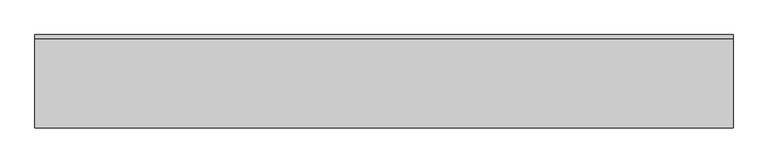
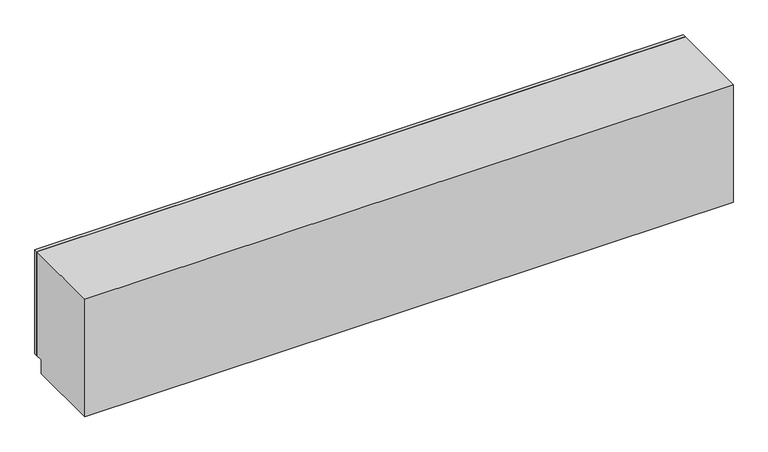
"""IFC4 building model written with IfcOpenShell, lengths in millimetres: furniture geometry, OD_CW_Base Cabinet : OD_CW_Base Cabinet."""

import ifcopenshell
import ifcopenshell.guid

model = None  # the IFC model being written
_history = None  # IfcOwnerHistory: only IFC2X3 demands one
_inside = {}  # id of a spatial element -> (the spatial element, [elements in it])
_under = {}  # id of a project, library or spatial element -> (it, [spatial elements below it])
_declared = {}  # id of a project -> (the project, [libraries it declares])
_typed = {}  # id of a type object -> (the type object, [elements of that type])
_made_of = {}  # id of a material, layer set ... -> (it, [elements and type objects made of it])


def new_model(schema):
    """Start an empty IFC model of exactly this schema.

    Asked for "IFC4X3", IfcOpenShell would pick the latest addendum, in which some entities
    have other attributes; the version numbers below select the first issue.
    IFC2X3 requires an IfcOwnerHistory on every rooted entity: one is made here for all.
    """
    global model, _history
    if schema == "IFC4X3":
        model = ifcopenshell.file(schema_version=(4, 3, 0, 0))
    else:
        model = ifcopenshell.file(schema=schema)
    _inside.clear()
    _under.clear()
    _declared.clear()
    _typed.clear()
    _made_of.clear()
    _history = None
    if model.schema == "IFC2X3":
        org = make("IfcOrganization", Name="unknown")
        user = make(
            "IfcPersonAndOrganization",
            ThePerson=make("IfcPerson", FamilyName="unknown"),
            TheOrganization=org,
        )
        app = make(
            "IfcApplication",
            ApplicationDeveloper=org,
            Version="unknown",
            ApplicationFullName="unknown",
            ApplicationIdentifier="unknown",
        )
        _history = make(
            "IfcOwnerHistory",
            OwningUser=user,
            OwningApplication=app,
            ChangeAction="ADDED",
            CreationDate=0,
        )
    return model


def make(cls, **values):
    """One entity of the class cls with the attributes given. An attribute that is None is left unset."""
    return model.create_entity(
        cls, **{name: value for name, value in values.items() if value is not None}
    )


def rooted(cls, **values):
    """An entity with a GlobalId (a new one), such as an element, a storey or a relation."""
    return make(cls, GlobalId=ifcopenshell.guid.new(), OwnerHistory=_history, **values)


def si_unit(unit_type, name, prefix=None):
    """IfcSIUnit, for example si_unit("LENGTHUNIT", "METRE", prefix="MILLI")."""
    return make("IfcSIUnit", UnitType=unit_type, Prefix=prefix, Name=name)


def assignment(units):
    """IfcUnitAssignment: the units of a project."""
    return None if units is None else make("IfcUnitAssignment", Units=units)


def point(xyz):
    """IfcCartesianPoint."""
    return None if xyz is None else make("IfcCartesianPoint", Coordinates=xyz)


def direction(xyz):
    """IfcDirection."""
    return None if xyz is None else make("IfcDirection", DirectionRatios=xyz)


def frame(location, z_axis=None, x_axis=None):
    """IfcAxis2Placement3D, a coordinate frame: its origin and axes. An axis left out is left unset."""
    return make(
        "IfcAxis2Placement3D",
        Location=point(location),
        Axis=direction(z_axis),
        RefDirection=direction(x_axis),
    )


def origin():
    """The frame at (0, 0, 0) with its axes left unset."""
    return frame((0.0, 0.0, 0.0))


def place(relative_to, where):
    """IfcLocalPlacement: puts the frame where relative to a parent placement (None: the world)."""
    return make(
        "IfcLocalPlacement", PlacementRelTo=relative_to, RelativePlacement=where
    )


def context(
    kind, dimensions, precision=None, world=None, true_north=None, identifier=None
):
    """IfcGeometricRepresentationContext, for example the 3D "Model" context."""
    return make(
        "IfcGeometricRepresentationContext",
        ContextIdentifier=identifier,
        ContextType=kind,
        CoordinateSpaceDimension=dimensions,
        Precision=precision,
        WorldCoordinateSystem=world,
        TrueNorth=true_north,
    )


def project(units=None, contexts=None):
    """IfcProject with its units and contexts."""
    return rooted(
        "IfcProject",
        Name="project",
        RepresentationContexts=contexts,
        UnitsInContext=assignment(units),
    )


def spatial(cls, under=None, at=None, **own):
    """A site, building, storey or space (cls), placed at a placement, below another one or the project."""
    s = rooted(cls, ObjectPlacement=at, **own)
    if under is not None:
        _under.setdefault(under.id(), (under, []))[1].append(s)
    return s


def polyline(points):
    """IfcPolyline through the points."""
    return make("IfcPolyline", Points=[point(p) for p in points])


def outline(outer, holes=None, kind="AREA"):
    """IfcArbitraryClosedProfileDef: a profile drawn as a closed curve; with holes, ...WithVoids."""
    if holes is None:
        return make("IfcArbitraryClosedProfileDef", ProfileType=kind, OuterCurve=outer)
    return make(
        "IfcArbitraryProfileDefWithVoids",
        ProfileType=kind,
        OuterCurve=outer,
        InnerCurves=holes,
    )


def extrude(swept, where, along, depth):
    """IfcExtrudedAreaSolid: the profile swept, set in the frame where, extruded along a direction by depth."""
    return make(
        "IfcExtrudedAreaSolid",
        SweptArea=swept,
        Position=where,
        ExtrudedDirection=direction(along),
        Depth=depth,
    )


def shape(context_of_items, identifier, shape_type, items):
    """IfcShapeRepresentation: the items that make up one representation, for example the "Body"."""
    return make(
        "IfcShapeRepresentation",
        ContextOfItems=context_of_items,
        RepresentationIdentifier=identifier,
        RepresentationType=shape_type,
        Items=items,
    )


def source(mapping_origin, context_of_items, identifier, shape_type, items):
    """IfcRepresentationMap: a shape defined once, which mapped items show again and again."""
    return make(
        "IfcRepresentationMap",
        MappingOrigin=mapping_origin,
        MappedRepresentation=shape(context_of_items, identifier, shape_type, items),
    )


def transform(
    local_origin,
    x_axis=None,
    y_axis=None,
    z_axis=None,
    scale=None,
    scale2=None,
    scale3=None,
    uniform=True,
):
    """IfcCartesianTransformationOperator3D, or its non-uniform kind. x_axis, y_axis, z_axis: its Axis1, 2, 3."""
    if uniform:
        return make(
            "IfcCartesianTransformationOperator3D",
            Axis1=direction(x_axis),
            Axis2=direction(y_axis),
            LocalOrigin=point(local_origin),
            Scale=scale,
            Axis3=direction(z_axis),
        )
    return make(
        "IfcCartesianTransformationOperator3DnonUniform",
        Axis1=direction(x_axis),
        Axis2=direction(y_axis),
        LocalOrigin=point(local_origin),
        Scale=scale,
        Axis3=direction(z_axis),
        Scale2=scale2,
        Scale3=scale3,
    )


def mapped(mapping_source, mapping_target):
    """IfcMappedItem: shows the shape of a source again, moved by a transform."""
    return make(
        "IfcMappedItem", MappingSource=mapping_source, MappingTarget=mapping_target
    )


def made_of(thing, what):
    """Note that an element or type object is made of a material, layer set ...; save() writes the relation."""
    if what is not None:
        _made_of.setdefault(what.id(), (what, []))[1].append(thing)
    return thing


def element(
    cls,
    number,
    at=None,
    inside=None,
    cuts=None,
    type_object=None,
    material=None,
    context=None,
    identifier="Body",
    shape_type=None,
    held_by="IfcProductDefinitionShape",
    body=None,
    shapes=None,
    **own,
):
    """One element of the class cls, such as IfcWall. Its Tag is "e" and its number.

    at: its placement. inside: the storey or other place that contains it. cuts: it is an
    opening in that element (IfcRelVoidsElement). A single representation is given by context,
    identifier, shape_type and body (its items); several are given by shapes. held_by: the class
    of the entity that holds the representations. save() writes the other relations.
    """
    e = rooted(cls, Tag="e%d" % number, ObjectPlacement=at, **own)
    if body is not None:
        shapes = [shape(context, identifier, shape_type, body)]
    if shapes is not None:
        e.Representation = make(held_by, Representations=shapes)
    if inside is not None:
        _inside.setdefault(inside.id(), (inside, []))[1].append(e)
    if cuts is not None:
        rooted(
            "IfcRelVoidsElement", RelatingBuildingElement=cuts, RelatedOpeningElement=e
        )
    if type_object is not None:
        _typed.setdefault(type_object.id(), (type_object, []))[1].append(e)
    return made_of(e, material)


def aggregate(whole, parts):
    """IfcRelAggregates: a whole, such as a stair, and the parts it consists of."""
    return rooted("IfcRelAggregates", RelatingObject=whole, RelatedObjects=parts)


def save(model, path):
    """Write the relations noted so far, then the file.

    IfcRelAggregates (storeys below a building ...), IfcRelContainedInSpatialStructure (elements
    in a storey), IfcRelDefinesByType, IfcRelAssociatesMaterial and IfcRelDeclares: one each for
    every whole, place, type object, material and project.
    """
    for whole, parts in _under.values():
        aggregate(whole, parts)
    for where, things in _inside.values():
        rooted(
            "IfcRelContainedInSpatialStructure",
            RelatedElements=things,
            RelatingStructure=where,
        )
    for kind, things in _typed.values():
        rooted("IfcRelDefinesByType", RelatedObjects=things, RelatingType=kind)
    for what, things in _made_of.values():
        rooted("IfcRelAssociatesMaterial", RelatedObjects=things, RelatingMaterial=what)
    for by, libraries in _declared.values():
        rooted("IfcRelDeclares", RelatingContext=by, RelatedDefinitions=libraries)
    model.write(path)


def furniture_fdb20c35(model_context):
    return source(origin(), model_context, "Body", "SweptSolid", [
        extrude(outline(polyline([(18.7377049, -25.4), (18.7377049, 0.0), (4581.8428379, 0.0), (4581.8428379, -25.4), (18.7377049, -25.4)])), frame((0.0, 0.0, 101.6), z_axis=(0.0, 0.0, 1.0), x_axis=(1.0, 0.0, 0.0)), (0.0, 0.0, 1.0), 774.7),
        extrude(outline(polyline([(-25.4, 876.3), (-25.4, 101.6), (-76.2, 101.6), (-76.2, 0.0), (-609.6, 0.0), (-609.6, 876.3), (-25.4, 876.3)])), frame((18.7377049, 0.0, 0.0), z_axis=(1.0, 0.0, 0.0), x_axis=(0.0, 1.0, 0.0)), (0.0, 0.0, 1.0), 4563.105133),
    ])


if __name__ == "__main__":
    model = new_model("IFC4")
    model_context = context("Model", 3, world=origin())
    ifc_project = project(units=[si_unit("LENGTHUNIT", "METRE", prefix="MILLI")], contexts=[model_context])
    site = spatial("IfcSite", under=ifc_project)
    building = spatial("IfcBuilding", under=site)
    placement = place(None, origin())
    furniture_shape = furniture_fdb20c35(model_context)
    element("IfcFurniture", 1, ObjectType="OD_CW_Base Cabinet : OD_CW_Base Cabinet", at=placement, inside=building, context=model_context, shape_type="MappedRepresentation", body=[
        mapped(furniture_shape, transform((0.0, 0.0, 0.0), x_axis=(1.0, 0.0, 0.0), y_axis=(0.0, 1.0, 0.0), z_axis=(0.0, 0.0, 1.0))),
    ])
    save(model, "model.ifc")

# Revit data of these elements
# Type "OD_CW_Base Cabinet : OD_CW_Base Cabinet"
#   OD_CW_Width [instance default] = 2' - 10"
#   OD_CW_Length [instance default] = 8' - 0"
#   OD_CW_Height [instance default] = 2' - 3"
#   Depth = 2' - 0"
#   Height = 3' - 0"
#   Width = 4' - 0"
#   OD_CW_Material_Front Panel [instance default] = none
#   OD_CW_Material_Body [instance default] = none
# Element 1 (IfcFurniture, "OD_CW_Base Cabinet : OD_CW_Base Cabinet")
#   OD_CW_Width = 2' - 0"
#   OD_CW_Length = 14' - 11.64981"
#   OD_CW_Height = 2' - 10 1/2"
